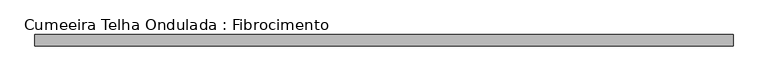
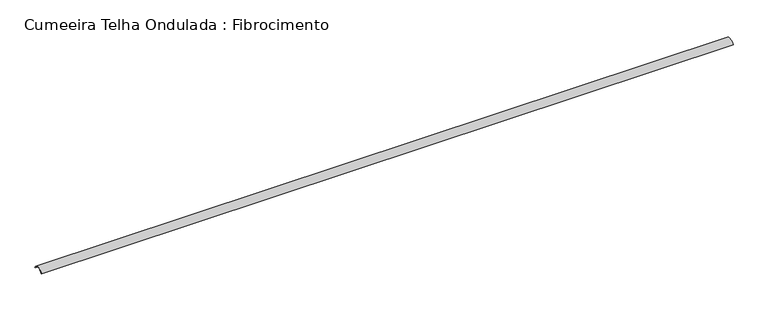
"""IFC4 building model written with IfcOpenShell, lengths in millimetres: beam geometry, Cumeeira Telha Ondulada : Fibrocimento."""

from ifc_helpers import new_model, si_unit, point, frame, frame_2d, origin, place, context, project, spatial, polyline, circle_curve, trimmed, segment, composite_curve, outline, extrude, source, transform, mapped, element, save


def cumeeira_telha_ondulada_fibrocimento_28917381(model_context):
    return source(origin(), model_context, "Body", "SweptSolid", [
        extrude(outline(composite_curve([segment(polyline([(58.3970135, 42.4437972), (53.9055884, 40.2467307)]), True, "CONTINUOUS"), segment(trimmed(circle_curve(frame_2d((-1.6029865, 13.0936483)), 61.7939461), [point((53.9055884, 40.2467307))], [point((-57.1115615, 40.2467307))], True, "CARTESIAN"), True, "CONTINUOUS"), segment(polyline([(-57.1115615, 40.2467307), (-61.6029865, 42.4437972)]), True, "CONTINUOUS"), segment(trimmed(circle_curve(frame_2d((-1.6029865, 13.0936483)), 66.7939461), [point((-61.6029865, 42.4437972))], [point((58.3970135, 42.4437972))], False, "CARTESIAN"), True, "CONTINUOUS")], self_intersect=False)), frame((-3626.5, 0.0, 0.0), z_axis=(1.0, 0.0, 0.0), x_axis=(0.0, 1.0, 0.0)), (0.0, 0.0, 1.0), 7253.0),
    ])


if __name__ == "__main__":
    model = new_model("IFC4")
    model_context = context("Model", 3, world=origin())
    ifc_project = project(units=[si_unit("LENGTHUNIT", "METRE", prefix="MILLI")], contexts=[model_context])
    site = spatial("IfcSite", under=ifc_project)
    building = spatial("IfcBuilding", under=site)
    placement = place(None, origin())
    cumeeira_telha_ondulada_fibrocimento_shape = cumeeira_telha_ondulada_fibrocimento_28917381(model_context)
    element("IfcBeam", 1, ObjectType="Cumeeira Telha Ondulada : Fibrocimento", at=placement, inside=building, context=model_context, shape_type="MappedRepresentation", body=[
        mapped(cumeeira_telha_ondulada_fibrocimento_shape, transform((0.0, 0.0, 0.0), x_axis=(1.0, 0.0, 0.0), y_axis=(0.0, 1.0, 0.0), z_axis=(0.0, 0.0, 1.0))),
    ])
    save(model, "model.ifc")

# Revit data of these elements
# Type "Cumeeira Telha Ondulada : Fibrocimento"
#   Cost = 5
#   Length [instance default] = 1.524 m
#   b = 0.07 m
#   h = 0.16 m
#   Structural Material = .TELHA DE FIBROCIMENTO
#   Assembly Code = ""
# Element 1 (IfcBeam, "Cumeeira Telha Ondulada : Fibrocimento")
#   Materials on its faces: ".TELHA DE FIBROCIMENTO"
# Materials
#   ".TELHA DE FIBROCIMENTO": class "CC_TELHADO", colour RGB 77 77 76, transparency 0, Description = "TELHA ONDULADA FIBROCIMENTO", Cost = 0
